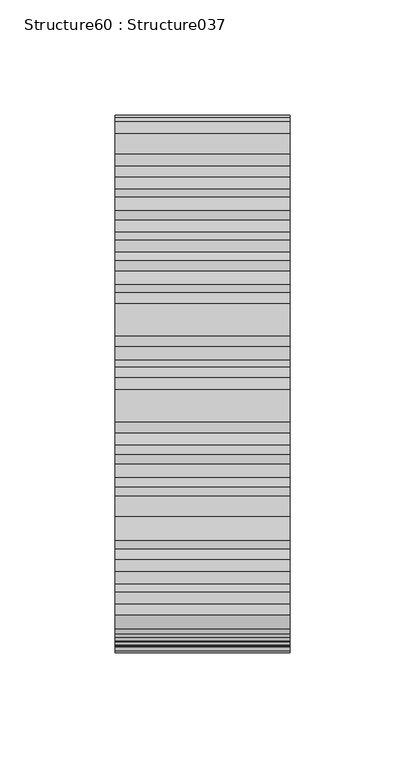
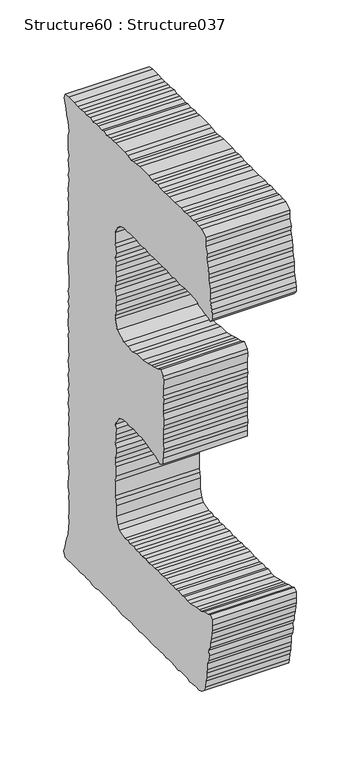
"""IFC4 building model written with IfcOpenShell, lengths in millimetres: proxy geometry, Structure60 : Structure037."""

from ifc_helpers import new_model, si_unit, frame, origin, place, context, project, spatial, polyline, outline, extrude, source, transform, mapped, element, save


def structure60_structure037_26cd2624(model_context):
    return source(origin(), model_context, "Body", "SweptSolid", [
        extrude(outline(polyline([(280152.5561884, 3552.242032), (280147.2802489, 3556.3417965), (280146.7058004, 3559.8671125), (280146.1137014, 3565.7094775), (280144.3550549, 3570.4109687), (280144.3550549, 3574.5107332), (280143.1885074, 3578.6104977), (280143.1885074, 3584.4689087), (280141.4298609, 3588.5702778), (280140.256895, 3593.8285667), (280140.8377618, 3598.5284533), (280138.4950392, 3602.6298224), (280139.0887429, 3606.7295868), (280137.3204687, 3611.4134274), (280136.7363927, 3617.2718384), (280135.5714498, 3620.7971545), (280135.5714498, 3625.472972), (280135.5714498, 3631.3410106), (280139.0887429, 3633.6821286), (280142.0139369, 3632.5155811), (280147.8707433, 3631.3410106), (280151.9721124, 3629.5984101), (280156.0718769, 3628.4158166), (280160.765345, 3627.8397636), (280170.1330261, 3625.472972), (280174.8248896, 3625.472972), (280179.5183578, 3626.6571701), (280183.0340462, 3625.472972), (280188.8844342, 3626.6571701), (280192.9858033, 3625.472972), (280197.6760622, 3626.0554434), (280201.7774313, 3625.472972), (280207.6358424, 3626.6571701), (280212.9117819, 3626.0554434), (280217.0115464, 3625.472972), (280221.1209385, 3626.6571701), (280226.3792275, 3625.472972), (280230.4886196, 3626.0554434), (280235.1708555, 3625.472972), (280239.8643236, 3626.6571701), (280245.7227347, 3625.472972), (280250.9986742, 3626.0554434), (280255.6889332, 3625.472972), (280259.2078308, 3626.6571701), (280265.0582188, 3625.472972), (280268.5755119, 3626.6571701), (280273.2577478, 3626.0554434), (280282.052585, 3628.4158166), (280284.3920984, 3631.915459), (280286.734821, 3638.9580681), (280286.734821, 3648.9258713), (280287.32692, 3654.1841602), (280287.9093915, 3657.7014533), (280287.9093915, 3671.7690209), (280287.32692, 3677.0449604), (280287.32692, 3685.8285655), (280287.9093915, 3689.3458585), (280287.9093915, 3694.029699), (280286.734821, 3699.3136616), (280286.734821, 3704.0135482), (280287.9093915, 3708.087639), (280287.32692, 3712.2146818), (280287.32692, 3716.8985223), (280286.734821, 3722.7312597), (280287.9093915, 3726.2742264), (280283.809627, 3733.8736333), (280282.052585, 3736.2163558), (280274.4419459, 3739.1592005), (280269.1563787, 3739.1592005), (280265.0582188, 3738.5574738), (280259.2078308, 3739.7416719), (280255.6889332, 3739.1592005), (280249.8241038, 3738.5574738), (280245.7227347, 3739.1592005), (280236.937525, 3737.400554), (280232.2472661, 3735.6146291), (280226.3792275, 3734.47536), (280222.2778584, 3733.2991849), (280218.1861169, 3730.9323932), (280212.3180783, 3734.47536), (280212.3180783, 3739.7416719), (280212.9117819, 3744.4158848), (280211.7372114, 3748.5429276), (280212.9117819, 3753.8012165), (280212.3180783, 3757.8753073), (280212.9117819, 3762.0023501), (280212.9117819, 3766.684586), (280211.7372114, 3771.3860772), (280211.7372114, 3776.6427615), (280212.9117819, 3781.9299333), (280212.3180783, 3785.4456218), (280212.9117819, 3791.3056374), (280211.7372114, 3795.960595), (280212.3180783, 3799.5051664), (280212.9117819, 3805.3459267), (280211.7372114, 3814.7296538), (280212.3180783, 3818.2309008), (280217.0115464, 3822.348316), (280221.70341, 3820.015221), (280226.9713265, 3818.8310229), (280231.0726956, 3817.6741031), (280236.937525, 3815.9154565), (280245.1306356, 3814.148787), (280254.5143627, 3814.148787), (280260.3647507, 3812.9726119), (280268.5755119, 3812.9726119), (280274.4419459, 3813.5743386), (280284.9841975, 3818.8310229), (280287.9093915, 3827.6162325), (280287.9093915, 3831.1575946), (280286.734821, 3835.8334121), (280287.32692, 3840.5172527), (280286.734821, 3845.8012153), (280286.734821, 3849.8753061), (280287.9093915, 3855.1769193), (280287.9093915, 3859.2606378), (280286.734821, 3863.9332461), (280286.734821, 3868.0618934), (280287.32692, 3873.3185778), (280287.32692, 3878.5784713), (280286.734821, 3883.2863809), (280287.9093915, 3886.2051565), (280286.734821, 3891.5067697), (280287.32692, 3896.763454), (280287.9093915, 3900.2887701), (280287.9093915, 3910.8310217), (280284.9841975, 3916.6653636), (280281.468509, 3920.7908018), (280273.8498469, 3923.7079727), (280268.5755119, 3923.1319197), (280263.8820437, 3923.7079727), (280254.5143627, 3923.7079727), (280250.9986742, 3923.1319197), (280245.1306356, 3922.5494483), (280241.0292665, 3923.7079727), (280235.7629546, 3922.5494483), (280231.6631901, 3922.5494483), (280226.9713265, 3923.1319197), (280212.9117819, 3923.1319197), (280207.0517663, 3923.7079727), (280202.3695304, 3922.5494483), (280198.2697659, 3922.5494483), (280193.5762978, 3923.7079727), (280188.8844342, 3922.5494483), (280183.6181223, 3922.5494483), (280179.5183578, 3923.7079727), (280170.1330261, 3923.7079727), (280159.5891699, 3922.5494483), (280156.6655805, 3920.2067257), (280151.9721124, 3919.6066036), (280147.2802489, 3918.4480792), (280142.0139369, 3917.8479571), (280139.0887429, 3915.5068392), (280135.5714498, 3919.6066036), (280135.5714498, 3924.2888396), (280136.1555259, 3928.4158823), (280137.9141724, 3933.6741713), (280138.4950392, 3937.1930689), (280139.0887429, 3942.4770315), (280139.0887429, 3946.5511223), (280140.256895, 3951.2606365), (280141.4298609, 3955.360401), (280140.8377618, 3959.4617701), (280142.0139369, 3965.3201811), (280143.7725834, 3969.994394), (280144.3550549, 3973.5197101), (280143.7725834, 3977.6194746), (280146.1137014, 3983.4794902), (280146.1137014, 3988.1633307), (280146.1137014, 3991.6806238), (280151.9721124, 3996.390138), (280156.6655805, 3996.390138), (280161.9399155, 3996.9645864), (280165.4572086, 3996.390138), (280170.7235205, 3996.9645864), (280176.0010647, 3996.9645864), (280180.6929283, 3995.7803883), (280184.2005937, 3996.9645864), (280194.7524729, 3995.7803883), (280203.5264502, 3995.7803883), (280207.6358424, 3996.390138), (280211.7372114, 3995.7803883), (280217.6052501, 3995.7803883), (280221.70341, 3996.9645864), (280225.8031745, 3996.9645864), (280231.0726956, 3995.7803883), (280235.7629546, 3996.9645864), (280249.8241038, 3996.9645864), (280255.0984387, 3996.390138), (280259.7806746, 3995.7803883), (280262.7171009, 3995.7803883), (280268.5755119, 3996.390138), (280273.2577478, 3996.9645864), (280287.32692, 3996.9645864), (280292.0091559, 3996.390138), (280295.526449, 3996.9645864), (280301.376837, 3995.7803883), (280306.0703051, 3996.9645864), (280309.5859936, 3995.7803883), (280314.8619332, 3996.390138), (280318.3776216, 3996.390138), (280323.6471428, 3995.7803883), (280327.7453027, 3996.9645864), (280333.6133413, 3995.7803883), (280337.1306344, 3996.390138), (280342.3985509, 3995.7803883), (280347.0807868, 3995.7803883), (280352.3647494, 3996.390138), (280361.1499591, 3996.390138), (280366.4258986, 3995.7803883), (280368.1829406, 3991.6806238), (280366.4258986, 3987.5792547), (280365.2513281, 3982.8793681), (280364.6576245, 3977.6194746), (280361.7324305, 3972.3627903), (280360.565883, 3964.1343784), (280361.7324305, 3958.8776941), (280361.7324305, 3945.9766739), (280360.565883, 3940.718385), (280361.7324305, 3935.4328178), (280361.1499591, 3931.9058971), (280360.565883, 3926.0490907), (280361.7324305, 3921.3748778), (280360.565883, 3917.8479571), (280361.7324305, 3907.3313793), (280361.1499591, 3902.6314927), (280361.7324305, 3897.9476522), (280361.1499591, 3894.4030808), (280361.1499591, 3889.7208449), (280361.7324305, 3884.4609514), (280361.1499591, 3879.7610648), (280361.7324305, 3874.5043805), (280360.565883, 3866.3032469), (280361.1499591, 3861.0192843), (280360.565883, 3855.7353217), (280360.565883, 3852.2340747), (280361.7324305, 3846.9757858), (280361.7324305, 3836.9919366), (280361.1499591, 3832.8921721), (280361.1499591, 3828.2163546), (280360.565883, 3824.1149855), (280360.565883, 3814.7296538), (280361.7324305, 3810.0474179), (280360.565883, 3804.7730829), (280361.7324305, 3799.5051664), (280360.565883, 3795.960595), (280361.7324305, 3791.3056374), (280361.1499591, 3786.6298199), (280361.7324305, 3781.3282066), (280361.7324305, 3777.2444882), (280360.565883, 3771.3860772), (280361.7324305, 3767.8607611), (280361.1499591, 3762.5848215), (280361.1499591, 3753.2171405), (280360.565883, 3748.5429276), (280361.7324305, 3743.2332913), (280361.1499591, 3739.1592005), (280360.565883, 3733.8736333), (280361.7324305, 3730.3563402), (280361.1499591, 3725.0996559), (280360.565883, 3720.4158154), (280361.7324305, 3715.1302482), (280360.565883, 3710.4560353), (280361.1499591, 3706.9130685), (280361.7324305, 3701.6547796), (280360.565883, 3696.3884676), (280361.1499591, 3692.2710525), (280360.565883, 3687.587212), (280361.1499591, 3682.8857208), (280360.565883, 3677.6274319), (280360.565883, 3672.9435914), (280361.1499591, 3668.8261762), (280361.1499591, 3663.5598643), (280360.565883, 3658.8840468), (280361.7324305, 3654.7842823), (280361.1499591, 3650.1004418), (280361.7324305, 3645.4262289), (280361.1499591, 3641.2991861), (280360.565883, 3636.0408972), (280361.1499591, 3630.7392839), (280361.7324305, 3626.6571701), (280361.7324305, 3621.3732075), (280360.565883, 3616.69739), (280361.1499591, 3612.0135494), (280360.565883, 3607.3393366), (280360.565883, 3597.9540049), (280361.1499591, 3593.8285667), (280360.565883, 3588.5702778), (280361.1499591, 3583.8864372), (280362.3149019, 3575.6853037), (280364.0831761, 3570.9854171), (280365.832195, 3565.7094775), (280366.4258986, 3561.6257591), (280369.349488, 3555.7416744), (280366.4258986, 3551.0658569), (280361.7324305, 3551.0658569), (280356.4661185, 3551.6675836), (280347.0807868, 3551.6675836), (280342.9794177, 3551.0658569), (280337.1306344, 3551.6675836), (280332.4387708, 3551.0658569), (280328.3374017, 3551.6675836), (280323.6471428, 3550.4833855), (280318.9616977, 3550.4833855), (280314.2778571, 3551.6675836), (280296.110525, 3551.6675836), (280291.4282891, 3551.0658569), (280287.32692, 3551.6675836), (280276.7750409, 3550.4833855), (280272.6736718, 3550.4833855), (280267.3993368, 3551.0658569), (280263.8820437, 3551.6675836), (280258.6157318, 3551.0658569), (280253.9222636, 3551.0658569), (280249.8241038, 3550.4833855), (280244.5561872, 3551.6675836), (280235.1708555, 3551.6675836), (280231.6631901, 3551.0658569), (280217.6052501, 3551.0658569), (280212.9117819, 3551.6675836), (280208.2199184, 3550.4833855), (280204.1201539, 3551.6675836), (280199.4347088, 3551.6675836), (280194.7524729, 3551.0658569), (280188.8844342, 3550.4833855), (280185.3671412, 3551.6675836), (280174.8248896, 3551.6675836), (280170.7235205, 3550.4833855), (280161.3478165, 3551.6675836), (280156.0718769, 3551.0658569), (280152.5561884, 3552.242032)])), frame((-59031.6926606, 0.0, 0.0), z_axis=(1.0, 0.0, 0.0), x_axis=(0.0, 1.0, 0.0)), (0.0, 0.0, 1.0), 76.2),
    ])


if __name__ == "__main__":
    model = new_model("IFC4")
    model_context = context("Model", 3, world=origin())
    ifc_project = project(units=[si_unit("LENGTHUNIT", "METRE", prefix="MILLI")], contexts=[model_context])
    site = spatial("IfcSite", under=ifc_project)
    building = spatial("IfcBuilding", under=site)
    placement = place(None, origin())
    structure60_structure037_shape = structure60_structure037_26cd2624(model_context)
    element("IfcBuildingElementProxy", 1, Name="Structure60 : Structure037", ObjectType="Structure60 : Structure037", at=placement, inside=building, context=model_context, shape_type="MappedRepresentation", body=[
        mapped(structure60_structure037_shape, transform((0.0, 0.0, 0.0), x_axis=(1.0, 0.0, 0.0), y_axis=(0.0, 1.0, 0.0), z_axis=(0.0, 0.0, 1.0))),
    ])
    save(model, "model.ifc")

# Revit data of these elements
# Type "Structure60 : Structure037"
#   NameOverride = "Structure037"
# Element 1 (IfcBuildingElementProxy, "Structure60 : Structure037")
#   Materials on its faces: "BRUSHED ALUM. LETTERING"
# Materials
#   "BRUSHED ALUM. LETTERING": class "Unassigned", colour RGB 169 181 186, transparency 0, Cost = 0
